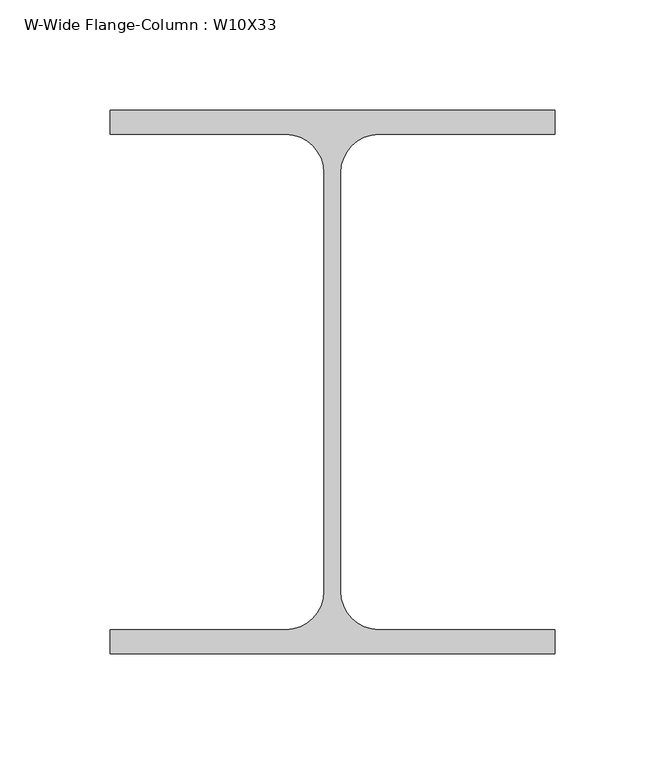
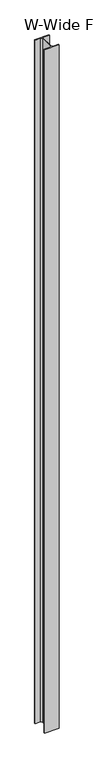
"""IFC4 building model written with IfcOpenShell, lengths in millimetres: column geometry, W-Wide Flange-Column : W10X33."""

import ifcopenshell
import ifcopenshell.guid

model = None  # the IFC model being written
_history = None  # IfcOwnerHistory: only IFC2X3 demands one
_inside = {}  # id of a spatial element -> (the spatial element, [elements in it])
_under = {}  # id of a project, library or spatial element -> (it, [spatial elements below it])
_declared = {}  # id of a project -> (the project, [libraries it declares])
_typed = {}  # id of a type object -> (the type object, [elements of that type])
_made_of = {}  # id of a material, layer set ... -> (it, [elements and type objects made of it])


def new_model(schema):
    """Start an empty IFC model of exactly this schema.

    Asked for "IFC4X3", IfcOpenShell would pick the latest addendum, in which some entities
    have other attributes; the version numbers below select the first issue.
    IFC2X3 requires an IfcOwnerHistory on every rooted entity: one is made here for all.
    """
    global model, _history
    if schema == "IFC4X3":
        model = ifcopenshell.file(schema_version=(4, 3, 0, 0))
    else:
        model = ifcopenshell.file(schema=schema)
    _inside.clear()
    _under.clear()
    _declared.clear()
    _typed.clear()
    _made_of.clear()
    _history = None
    if model.schema == "IFC2X3":
        org = make("IfcOrganization", Name="unknown")
        user = make(
            "IfcPersonAndOrganization",
            ThePerson=make("IfcPerson", FamilyName="unknown"),
            TheOrganization=org,
        )
        app = make(
            "IfcApplication",
            ApplicationDeveloper=org,
            Version="unknown",
            ApplicationFullName="unknown",
            ApplicationIdentifier="unknown",
        )
        _history = make(
            "IfcOwnerHistory",
            OwningUser=user,
            OwningApplication=app,
            ChangeAction="ADDED",
            CreationDate=0,
        )
    return model


def make(cls, **values):
    """One entity of the class cls with the attributes given. An attribute that is None is left unset."""
    return model.create_entity(
        cls, **{name: value for name, value in values.items() if value is not None}
    )


def rooted(cls, **values):
    """An entity with a GlobalId (a new one), such as an element, a storey or a relation."""
    return make(cls, GlobalId=ifcopenshell.guid.new(), OwnerHistory=_history, **values)


def si_unit(unit_type, name, prefix=None):
    """IfcSIUnit, for example si_unit("LENGTHUNIT", "METRE", prefix="MILLI")."""
    return make("IfcSIUnit", UnitType=unit_type, Prefix=prefix, Name=name)


def assignment(units):
    """IfcUnitAssignment: the units of a project."""
    return None if units is None else make("IfcUnitAssignment", Units=units)


def point(xyz):
    """IfcCartesianPoint."""
    return None if xyz is None else make("IfcCartesianPoint", Coordinates=xyz)


def direction(xyz):
    """IfcDirection."""
    return None if xyz is None else make("IfcDirection", DirectionRatios=xyz)


def frame(location, z_axis=None, x_axis=None):
    """IfcAxis2Placement3D, a coordinate frame: its origin and axes. An axis left out is left unset."""
    return make(
        "IfcAxis2Placement3D",
        Location=point(location),
        Axis=direction(z_axis),
        RefDirection=direction(x_axis),
    )


def frame_2d(location, x_axis=None):
    """IfcAxis2Placement2D, a coordinate frame in the plane: its origin and x axis."""
    return make(
        "IfcAxis2Placement2D", Location=point(location), RefDirection=direction(x_axis)
    )


def origin():
    """The frame at (0, 0, 0) with its axes left unset."""
    return frame((0.0, 0.0, 0.0))


def place(relative_to, where):
    """IfcLocalPlacement: puts the frame where relative to a parent placement (None: the world)."""
    return make(
        "IfcLocalPlacement", PlacementRelTo=relative_to, RelativePlacement=where
    )


def context(
    kind, dimensions, precision=None, world=None, true_north=None, identifier=None
):
    """IfcGeometricRepresentationContext, for example the 3D "Model" context."""
    return make(
        "IfcGeometricRepresentationContext",
        ContextIdentifier=identifier,
        ContextType=kind,
        CoordinateSpaceDimension=dimensions,
        Precision=precision,
        WorldCoordinateSystem=world,
        TrueNorth=true_north,
    )


def project(units=None, contexts=None):
    """IfcProject with its units and contexts."""
    return rooted(
        "IfcProject",
        Name="project",
        RepresentationContexts=contexts,
        UnitsInContext=assignment(units),
    )


def spatial(cls, under=None, at=None, **own):
    """A site, building, storey or space (cls), placed at a placement, below another one or the project."""
    s = rooted(cls, ObjectPlacement=at, **own)
    if under is not None:
        _under.setdefault(under.id(), (under, []))[1].append(s)
    return s


def polyline(points):
    """IfcPolyline through the points."""
    return make("IfcPolyline", Points=[point(p) for p in points])


def circle_curve(where, radius):
    """IfcCircle in the frame where."""
    return make("IfcCircle", Position=where, Radius=radius)


def trimmed(basis, trim1, trim2, sense, master):
    """IfcTrimmedCurve: the piece of a basis curve between two trims."""
    return make(
        "IfcTrimmedCurve",
        BasisCurve=basis,
        Trim1=trim1,
        Trim2=trim2,
        SenseAgreement=sense,
        MasterRepresentation=master,
    )


def segment(curve, same_sense, transition):
    """IfcCompositeCurveSegment."""
    return make(
        "IfcCompositeCurveSegment",
        Transition=transition,
        SameSense=same_sense,
        ParentCurve=curve,
    )


def composite_curve(segments, self_intersect=None):
    """IfcCompositeCurve: segments joined end to end."""
    return make("IfcCompositeCurve", Segments=segments, SelfIntersect=self_intersect)


def outline(outer, holes=None, kind="AREA"):
    """IfcArbitraryClosedProfileDef: a profile drawn as a closed curve; with holes, ...WithVoids."""
    if holes is None:
        return make("IfcArbitraryClosedProfileDef", ProfileType=kind, OuterCurve=outer)
    return make(
        "IfcArbitraryProfileDefWithVoids",
        ProfileType=kind,
        OuterCurve=outer,
        InnerCurves=holes,
    )


def extrude(swept, where, along, depth):
    """IfcExtrudedAreaSolid: the profile swept, set in the frame where, extruded along a direction by depth."""
    return make(
        "IfcExtrudedAreaSolid",
        SweptArea=swept,
        Position=where,
        ExtrudedDirection=direction(along),
        Depth=depth,
    )


def shape(context_of_items, identifier, shape_type, items):
    """IfcShapeRepresentation: the items that make up one representation, for example the "Body"."""
    return make(
        "IfcShapeRepresentation",
        ContextOfItems=context_of_items,
        RepresentationIdentifier=identifier,
        RepresentationType=shape_type,
        Items=items,
    )


def source(mapping_origin, context_of_items, identifier, shape_type, items):
    """IfcRepresentationMap: a shape defined once, which mapped items show again and again."""
    return make(
        "IfcRepresentationMap",
        MappingOrigin=mapping_origin,
        MappedRepresentation=shape(context_of_items, identifier, shape_type, items),
    )


def transform(
    local_origin,
    x_axis=None,
    y_axis=None,
    z_axis=None,
    scale=None,
    scale2=None,
    scale3=None,
    uniform=True,
):
    """IfcCartesianTransformationOperator3D, or its non-uniform kind. x_axis, y_axis, z_axis: its Axis1, 2, 3."""
    if uniform:
        return make(
            "IfcCartesianTransformationOperator3D",
            Axis1=direction(x_axis),
            Axis2=direction(y_axis),
            LocalOrigin=point(local_origin),
            Scale=scale,
            Axis3=direction(z_axis),
        )
    return make(
        "IfcCartesianTransformationOperator3DnonUniform",
        Axis1=direction(x_axis),
        Axis2=direction(y_axis),
        LocalOrigin=point(local_origin),
        Scale=scale,
        Axis3=direction(z_axis),
        Scale2=scale2,
        Scale3=scale3,
    )


def mapped(mapping_source, mapping_target):
    """IfcMappedItem: shows the shape of a source again, moved by a transform."""
    return make(
        "IfcMappedItem", MappingSource=mapping_source, MappingTarget=mapping_target
    )


def made_of(thing, what):
    """Note that an element or type object is made of a material, layer set ...; save() writes the relation."""
    if what is not None:
        _made_of.setdefault(what.id(), (what, []))[1].append(thing)
    return thing


def element(
    cls,
    number,
    at=None,
    inside=None,
    cuts=None,
    type_object=None,
    material=None,
    context=None,
    identifier="Body",
    shape_type=None,
    held_by="IfcProductDefinitionShape",
    body=None,
    shapes=None,
    **own,
):
    """One element of the class cls, such as IfcWall. Its Tag is "e" and its number.

    at: its placement. inside: the storey or other place that contains it. cuts: it is an
    opening in that element (IfcRelVoidsElement). A single representation is given by context,
    identifier, shape_type and body (its items); several are given by shapes. held_by: the class
    of the entity that holds the representations. save() writes the other relations.
    """
    e = rooted(cls, Tag="e%d" % number, ObjectPlacement=at, **own)
    if body is not None:
        shapes = [shape(context, identifier, shape_type, body)]
    if shapes is not None:
        e.Representation = make(held_by, Representations=shapes)
    if inside is not None:
        _inside.setdefault(inside.id(), (inside, []))[1].append(e)
    if cuts is not None:
        rooted(
            "IfcRelVoidsElement", RelatingBuildingElement=cuts, RelatedOpeningElement=e
        )
    if type_object is not None:
        _typed.setdefault(type_object.id(), (type_object, []))[1].append(e)
    return made_of(e, material)


def aggregate(whole, parts):
    """IfcRelAggregates: a whole, such as a stair, and the parts it consists of."""
    return rooted("IfcRelAggregates", RelatingObject=whole, RelatedObjects=parts)


def save(model, path):
    """Write the relations noted so far, then the file.

    IfcRelAggregates (storeys below a building ...), IfcRelContainedInSpatialStructure (elements
    in a storey), IfcRelDefinesByType, IfcRelAssociatesMaterial and IfcRelDeclares: one each for
    every whole, place, type object, material and project.
    """
    for whole, parts in _under.values():
        aggregate(whole, parts)
    for where, things in _inside.values():
        rooted(
            "IfcRelContainedInSpatialStructure",
            RelatedElements=things,
            RelatingStructure=where,
        )
    for kind, things in _typed.values():
        rooted("IfcRelDefinesByType", RelatedObjects=things, RelatingType=kind)
    for what, things in _made_of.values():
        rooted("IfcRelAssociatesMaterial", RelatedObjects=things, RelatingMaterial=what)
    for by, libraries in _declared.values():
        rooted("IfcRelDeclares", RelatingContext=by, RelatedDefinitions=libraries)
    model.write(path)


def w_wide_flange_column_w10x33_0f134691(model_context):
    return source(origin(), model_context, "Body", "SweptSolid", [
        extrude(outline(composite_curve([segment(polyline([(101.092, 123.571), (101.092, 112.522), (21.209, 112.522)]), True, "CONTINUOUS"), segment(trimmed(circle_curve(frame_2d((21.209, 94.996)), 17.526), [point((21.209, 112.522))], [point((3.683, 94.996))], True, "CARTESIAN"), True, "CONTINUOUS"), segment(polyline([(3.683, 94.996), (3.683, -94.996)]), True, "CONTINUOUS"), segment(trimmed(circle_curve(frame_2d((21.209, -94.996)), 17.526), [point((3.683, -94.996))], [point((21.209, -112.522))], True, "CARTESIAN"), True, "CONTINUOUS"), segment(polyline([(21.209, -112.522), (101.092, -112.522), (101.092, -123.571), (-101.092, -123.571), (-101.092, -112.522), (-21.209, -112.522)]), True, "CONTINUOUS"), segment(trimmed(circle_curve(frame_2d((-21.209, -94.996)), 17.526), [point((-21.209, -112.522))], [point((-3.683, -94.996))], True, "CARTESIAN"), True, "CONTINUOUS"), segment(polyline([(-3.683, -94.996), (-3.683, 94.996)]), True, "CONTINUOUS"), segment(trimmed(circle_curve(frame_2d((-21.209, 94.996)), 17.526), [point((-3.683, 94.996))], [point((-21.209, 112.522))], True, "CARTESIAN"), True, "CONTINUOUS"), segment(polyline([(-21.209, 112.522), (-101.092, 112.522), (-101.092, 123.571), (101.092, 123.571)]), True, "CONTINUOUS")], self_intersect=False)), frame((0.0, 0.0, 8756.65), z_axis=(0.0, 0.0, 1.0), x_axis=(1.0, 0.0, 0.0)), (0.0, 0.0, 1.0), 10293.35),
    ])


if __name__ == "__main__":
    model = new_model("IFC4")
    model_context = context("Model", 3, world=origin())
    ifc_project = project(units=[si_unit("LENGTHUNIT", "METRE", prefix="MILLI")], contexts=[model_context])
    site = spatial("IfcSite", under=ifc_project)
    building = spatial("IfcBuilding", under=site)
    placement = place(None, origin())
    w_wide_flange_column_w10x33_shape = w_wide_flange_column_w10x33_0f134691(model_context)
    element("IfcColumn", 1, ObjectType="W-Wide Flange-Column : W10X33", at=placement, inside=building, context=model_context, shape_type="MappedRepresentation", body=[
        mapped(w_wide_flange_column_w10x33_shape, transform((0.0, 0.0, 0.0), x_axis=(1.0, 0.0, 0.0), y_axis=(0.0, 1.0, 0.0), z_axis=(0.0, 0.0, 1.0))),
    ])
    save(model, "model.ifc")

# Revit data of these elements
# Type "W-Wide Flange-Column : W10X33"
#   Assembly Code = "B10"
#   W = 33
#   bf = 0' - 7.96"
#   d = 0' - 9.73"
#   k = 0' - 1 1/8"
#   kr = 0' - 0.69"
#   tf = 0' - 0.435"
#   tw = 0' - 0.29"
#   A = 0.0674306 SF
#   Structural Material [instance default] = Steel ASTM A992
# Element 1 (IfcColumn, "W-Wide Flange-Column : W10X33")
#   Materials on its faces: "Steel ASTM A992"
# Materials
#   "Steel ASTM A992": class "Metal", colour RGB 199 199 199, transparency 0, Description = "Structural steel 50ksi", Cost = 0
